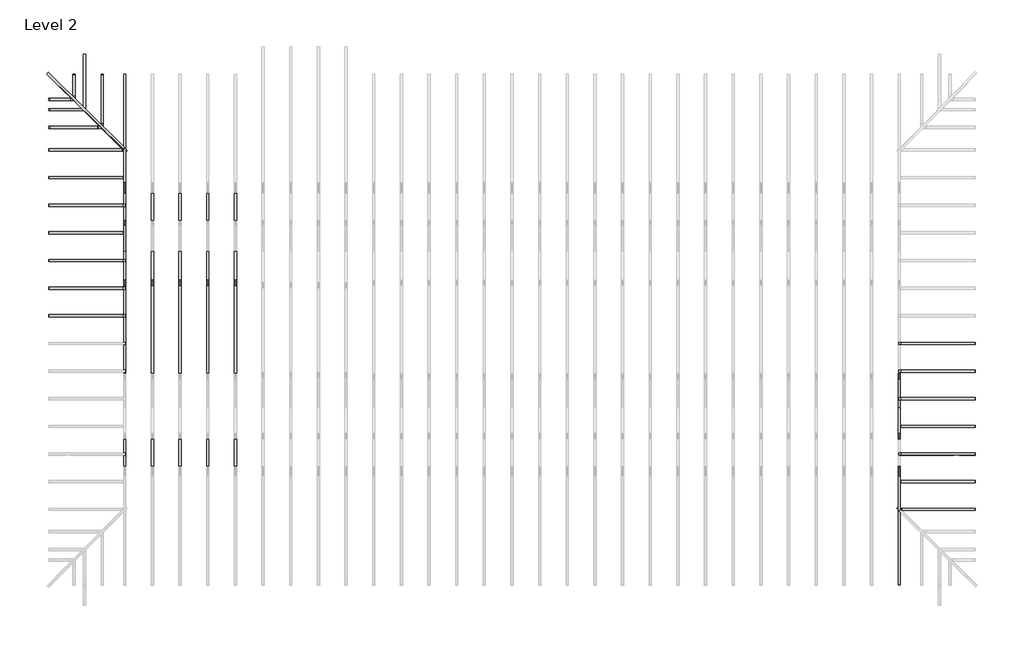
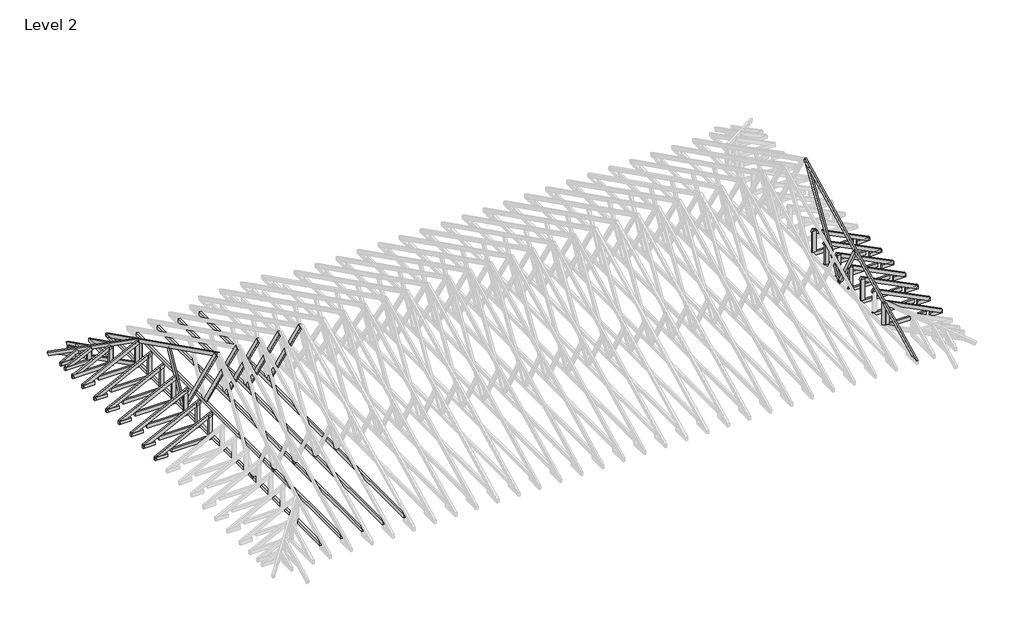
# One storey, part 3 of 5: 93 beams.
# Revit data of these elements (continued)
# Elements 24, 25, 26, 27, 28, 29, 30, 44, 81, 82, 83, 84, 85, 86, 87 (IfcBeam, "Dimension Lumber : BLDG 6241 2X4\" TRUSS MEMBER")
#   Comments = ""
#   Structural Material = Softwood, Lumber
#   Phase Created = New Construction
#   Materials on its faces: "Softwood, Lumber"
# Materials
#   "Softwood, Lumber": class "Wood", colour RGB 223 192 134, transparency 0, Description = "Pinus Echinata", Cost = 0
